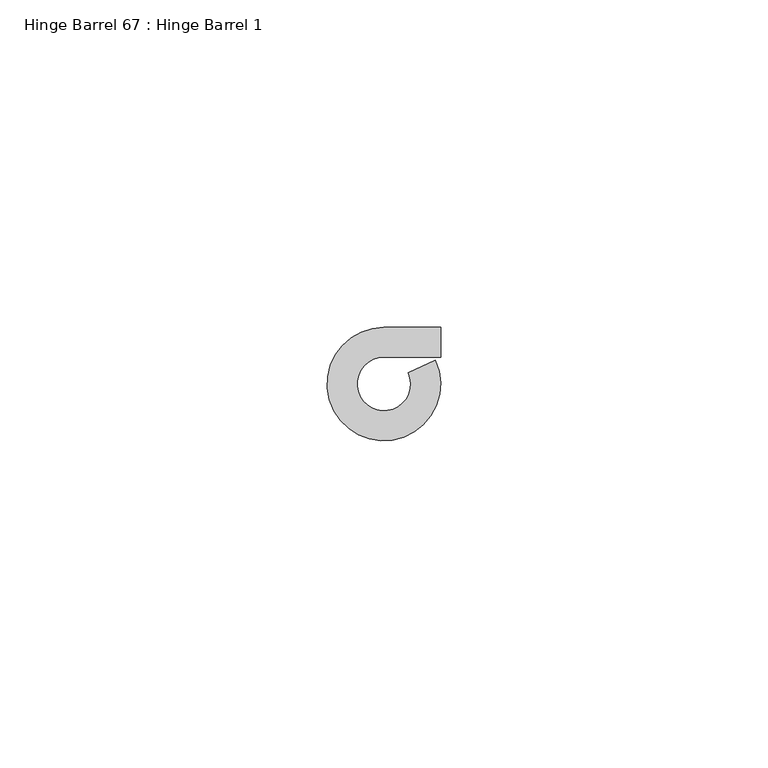
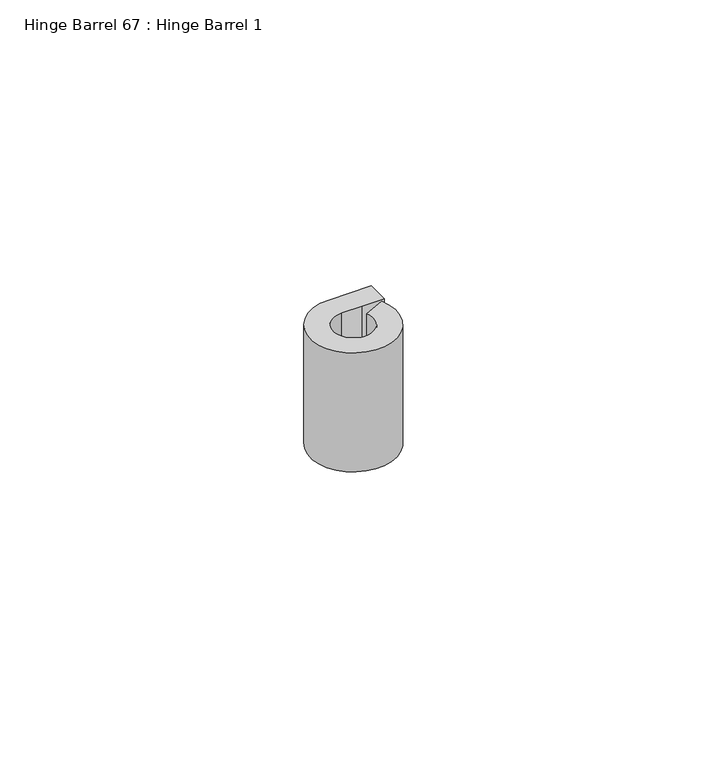
"""IFC4 building model written with IfcOpenShell, lengths in millimetres: proxy geometry, Hinge Barrel 67 : Hinge Barrel 1."""

import ifcopenshell
import ifcopenshell.guid

model = None  # the IFC model being written
_history = None  # IfcOwnerHistory: only IFC2X3 demands one
_inside = {}  # id of a spatial element -> (the spatial element, [elements in it])
_under = {}  # id of a project, library or spatial element -> (it, [spatial elements below it])
_declared = {}  # id of a project -> (the project, [libraries it declares])
_typed = {}  # id of a type object -> (the type object, [elements of that type])
_made_of = {}  # id of a material, layer set ... -> (it, [elements and type objects made of it])


def new_model(schema):
    """Start an empty IFC model of exactly this schema.

    Asked for "IFC4X3", IfcOpenShell would pick the latest addendum, in which some entities
    have other attributes; the version numbers below select the first issue.
    IFC2X3 requires an IfcOwnerHistory on every rooted entity: one is made here for all.
    """
    global model, _history
    if schema == "IFC4X3":
        model = ifcopenshell.file(schema_version=(4, 3, 0, 0))
    else:
        model = ifcopenshell.file(schema=schema)
    _inside.clear()
    _under.clear()
    _declared.clear()
    _typed.clear()
    _made_of.clear()
    _history = None
    if model.schema == "IFC2X3":
        org = make("IfcOrganization", Name="unknown")
        user = make(
            "IfcPersonAndOrganization",
            ThePerson=make("IfcPerson", FamilyName="unknown"),
            TheOrganization=org,
        )
        app = make(
            "IfcApplication",
            ApplicationDeveloper=org,
            Version="unknown",
            ApplicationFullName="unknown",
            ApplicationIdentifier="unknown",
        )
        _history = make(
            "IfcOwnerHistory",
            OwningUser=user,
            OwningApplication=app,
            ChangeAction="ADDED",
            CreationDate=0,
        )
    return model


def make(cls, **values):
    """One entity of the class cls with the attributes given. An attribute that is None is left unset."""
    return model.create_entity(
        cls, **{name: value for name, value in values.items() if value is not None}
    )


def rooted(cls, **values):
    """An entity with a GlobalId (a new one), such as an element, a storey or a relation."""
    return make(cls, GlobalId=ifcopenshell.guid.new(), OwnerHistory=_history, **values)


def si_unit(unit_type, name, prefix=None):
    """IfcSIUnit, for example si_unit("LENGTHUNIT", "METRE", prefix="MILLI")."""
    return make("IfcSIUnit", UnitType=unit_type, Prefix=prefix, Name=name)


def assignment(units):
    """IfcUnitAssignment: the units of a project."""
    return None if units is None else make("IfcUnitAssignment", Units=units)


def point(xyz):
    """IfcCartesianPoint."""
    return None if xyz is None else make("IfcCartesianPoint", Coordinates=xyz)


def direction(xyz):
    """IfcDirection."""
    return None if xyz is None else make("IfcDirection", DirectionRatios=xyz)


def frame(location, z_axis=None, x_axis=None):
    """IfcAxis2Placement3D, a coordinate frame: its origin and axes. An axis left out is left unset."""
    return make(
        "IfcAxis2Placement3D",
        Location=point(location),
        Axis=direction(z_axis),
        RefDirection=direction(x_axis),
    )


def frame_2d(location, x_axis=None):
    """IfcAxis2Placement2D, a coordinate frame in the plane: its origin and x axis."""
    return make(
        "IfcAxis2Placement2D", Location=point(location), RefDirection=direction(x_axis)
    )


def origin():
    """The frame at (0, 0, 0) with its axes left unset."""
    return frame((0.0, 0.0, 0.0))


def place(relative_to, where):
    """IfcLocalPlacement: puts the frame where relative to a parent placement (None: the world)."""
    return make(
        "IfcLocalPlacement", PlacementRelTo=relative_to, RelativePlacement=where
    )


def context(
    kind, dimensions, precision=None, world=None, true_north=None, identifier=None
):
    """IfcGeometricRepresentationContext, for example the 3D "Model" context."""
    return make(
        "IfcGeometricRepresentationContext",
        ContextIdentifier=identifier,
        ContextType=kind,
        CoordinateSpaceDimension=dimensions,
        Precision=precision,
        WorldCoordinateSystem=world,
        TrueNorth=true_north,
    )


def project(units=None, contexts=None):
    """IfcProject with its units and contexts."""
    return rooted(
        "IfcProject",
        Name="project",
        RepresentationContexts=contexts,
        UnitsInContext=assignment(units),
    )


def spatial(cls, under=None, at=None, **own):
    """A site, building, storey or space (cls), placed at a placement, below another one or the project."""
    s = rooted(cls, ObjectPlacement=at, **own)
    if under is not None:
        _under.setdefault(under.id(), (under, []))[1].append(s)
    return s


def polyline(points):
    """IfcPolyline through the points."""
    return make("IfcPolyline", Points=[point(p) for p in points])


def circle_curve(where, radius):
    """IfcCircle in the frame where."""
    return make("IfcCircle", Position=where, Radius=radius)


def trimmed(basis, trim1, trim2, sense, master):
    """IfcTrimmedCurve: the piece of a basis curve between two trims."""
    return make(
        "IfcTrimmedCurve",
        BasisCurve=basis,
        Trim1=trim1,
        Trim2=trim2,
        SenseAgreement=sense,
        MasterRepresentation=master,
    )


def segment(curve, same_sense, transition):
    """IfcCompositeCurveSegment."""
    return make(
        "IfcCompositeCurveSegment",
        Transition=transition,
        SameSense=same_sense,
        ParentCurve=curve,
    )


def composite_curve(segments, self_intersect=None):
    """IfcCompositeCurve: segments joined end to end."""
    return make("IfcCompositeCurve", Segments=segments, SelfIntersect=self_intersect)


def outline(outer, holes=None, kind="AREA"):
    """IfcArbitraryClosedProfileDef: a profile drawn as a closed curve; with holes, ...WithVoids."""
    if holes is None:
        return make("IfcArbitraryClosedProfileDef", ProfileType=kind, OuterCurve=outer)
    return make(
        "IfcArbitraryProfileDefWithVoids",
        ProfileType=kind,
        OuterCurve=outer,
        InnerCurves=holes,
    )


def extrude(swept, where, along, depth):
    """IfcExtrudedAreaSolid: the profile swept, set in the frame where, extruded along a direction by depth."""
    return make(
        "IfcExtrudedAreaSolid",
        SweptArea=swept,
        Position=where,
        ExtrudedDirection=direction(along),
        Depth=depth,
    )


def shape(context_of_items, identifier, shape_type, items):
    """IfcShapeRepresentation: the items that make up one representation, for example the "Body"."""
    return make(
        "IfcShapeRepresentation",
        ContextOfItems=context_of_items,
        RepresentationIdentifier=identifier,
        RepresentationType=shape_type,
        Items=items,
    )


def source(mapping_origin, context_of_items, identifier, shape_type, items):
    """IfcRepresentationMap: a shape defined once, which mapped items show again and again."""
    return make(
        "IfcRepresentationMap",
        MappingOrigin=mapping_origin,
        MappedRepresentation=shape(context_of_items, identifier, shape_type, items),
    )


def transform(
    local_origin,
    x_axis=None,
    y_axis=None,
    z_axis=None,
    scale=None,
    scale2=None,
    scale3=None,
    uniform=True,
):
    """IfcCartesianTransformationOperator3D, or its non-uniform kind. x_axis, y_axis, z_axis: its Axis1, 2, 3."""
    if uniform:
        return make(
            "IfcCartesianTransformationOperator3D",
            Axis1=direction(x_axis),
            Axis2=direction(y_axis),
            LocalOrigin=point(local_origin),
            Scale=scale,
            Axis3=direction(z_axis),
        )
    return make(
        "IfcCartesianTransformationOperator3DnonUniform",
        Axis1=direction(x_axis),
        Axis2=direction(y_axis),
        LocalOrigin=point(local_origin),
        Scale=scale,
        Axis3=direction(z_axis),
        Scale2=scale2,
        Scale3=scale3,
    )


def mapped(mapping_source, mapping_target):
    """IfcMappedItem: shows the shape of a source again, moved by a transform."""
    return make(
        "IfcMappedItem", MappingSource=mapping_source, MappingTarget=mapping_target
    )


def made_of(thing, what):
    """Note that an element or type object is made of a material, layer set ...; save() writes the relation."""
    if what is not None:
        _made_of.setdefault(what.id(), (what, []))[1].append(thing)
    return thing


def element(
    cls,
    number,
    at=None,
    inside=None,
    cuts=None,
    type_object=None,
    material=None,
    context=None,
    identifier="Body",
    shape_type=None,
    held_by="IfcProductDefinitionShape",
    body=None,
    shapes=None,
    **own,
):
    """One element of the class cls, such as IfcWall. Its Tag is "e" and its number.

    at: its placement. inside: the storey or other place that contains it. cuts: it is an
    opening in that element (IfcRelVoidsElement). A single representation is given by context,
    identifier, shape_type and body (its items); several are given by shapes. held_by: the class
    of the entity that holds the representations. save() writes the other relations.
    """
    e = rooted(cls, Tag="e%d" % number, ObjectPlacement=at, **own)
    if body is not None:
        shapes = [shape(context, identifier, shape_type, body)]
    if shapes is not None:
        e.Representation = make(held_by, Representations=shapes)
    if inside is not None:
        _inside.setdefault(inside.id(), (inside, []))[1].append(e)
    if cuts is not None:
        rooted(
            "IfcRelVoidsElement", RelatingBuildingElement=cuts, RelatedOpeningElement=e
        )
    if type_object is not None:
        _typed.setdefault(type_object.id(), (type_object, []))[1].append(e)
    return made_of(e, material)


def aggregate(whole, parts):
    """IfcRelAggregates: a whole, such as a stair, and the parts it consists of."""
    return rooted("IfcRelAggregates", RelatingObject=whole, RelatedObjects=parts)


def save(model, path):
    """Write the relations noted so far, then the file.

    IfcRelAggregates (storeys below a building ...), IfcRelContainedInSpatialStructure (elements
    in a storey), IfcRelDefinesByType, IfcRelAssociatesMaterial and IfcRelDeclares: one each for
    every whole, place, type object, material and project.
    """
    for whole, parts in _under.values():
        aggregate(whole, parts)
    for where, things in _inside.values():
        rooted(
            "IfcRelContainedInSpatialStructure",
            RelatedElements=things,
            RelatingStructure=where,
        )
    for kind, things in _typed.values():
        rooted("IfcRelDefinesByType", RelatedObjects=things, RelatingType=kind)
    for what, things in _made_of.values():
        rooted("IfcRelAssociatesMaterial", RelatedObjects=things, RelatingMaterial=what)
    for by, libraries in _declared.values():
        rooted("IfcRelDeclares", RelatingContext=by, RelatedDefinitions=libraries)
    model.write(path)


def hinge_barrel_67_hinge_barrel_1_2f8cd32d(model_context):
    return source(origin(), model_context, "Body", "SweptSolid", [
        extrude(outline(composite_curve([segment(polyline([(587323.2214739, -536306.2758841), (587319.1320739, -536306.2758841)]), True, "CONTINUOUS"), segment(trimmed(circle_curve(frame_2d((587319.1320739, -536310.3652841)), 4.0894), [point((587319.1320739, -536306.2758841))], [point((587322.8436736, -536308.6485371))], True, "CARTESIAN"), True, "CONTINUOUS"), segment(polyline([(587322.8436736, -536308.6485371), (587326.986084, -536306.7325249)]), True, "CONTINUOUS"), segment(trimmed(circle_curve(frame_2d((587319.1320739, -536310.3652841)), 8.6534625), [point((587326.986084, -536306.7325249))], [point((587319.1320739, -536301.7118216))], False, "CARTESIAN"), True, "CONTINUOUS"), segment(polyline([(587319.1320739, -536301.7118216), (587327.7934739, -536301.7118216), (587327.7934739, -536306.2758841), (587323.2214739, -536306.2758841)]), True, "CONTINUOUS")], self_intersect=False)), frame((0.0, 0.0, 1123.95), z_axis=(0.0, 0.0, 1.0), x_axis=(1.0, 0.0, 0.0)), (0.0, 0.0, 1.0), 25.4),
    ])


if __name__ == "__main__":
    model = new_model("IFC4")
    model_context = context("Model", 3, world=origin())
    ifc_project = project(units=[si_unit("LENGTHUNIT", "METRE", prefix="MILLI")], contexts=[model_context])
    site = spatial("IfcSite", under=ifc_project)
    building = spatial("IfcBuilding", under=site)
    placement = place(None, origin())
    hinge_barrel_67_hinge_barrel_1_shape = hinge_barrel_67_hinge_barrel_1_2f8cd32d(model_context)
    element("IfcBuildingElementProxy", 1, Name="Hinge Barrel 67 : Hinge Barrel 1", ObjectType="Hinge Barrel 67 : Hinge Barrel 1", at=placement, inside=building, context=model_context, shape_type="MappedRepresentation", body=[
        mapped(hinge_barrel_67_hinge_barrel_1_shape, transform((0.0, 0.0, 0.0), x_axis=(1.0, 0.0, 0.0), y_axis=(0.0, 1.0, 0.0), z_axis=(0.0, 0.0, 1.0))),
    ])
    save(model, "model.ifc")

# Revit data of these elements
# Element 1 (IfcBuildingElementProxy, "Hinge Barrel 67 : Hinge Barrel 1")
#   Materials on its faces: "6\"X6\" WELD-ON STL BUTT HINGE"
# Materials
#   "6\"X6\" WELD-ON STL BUTT HINGE": class "Metal", colour RGB 189 187 185, transparency 0, Description = "Carbon steel", Cost = 0
